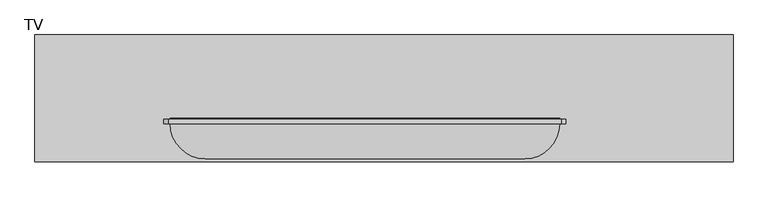
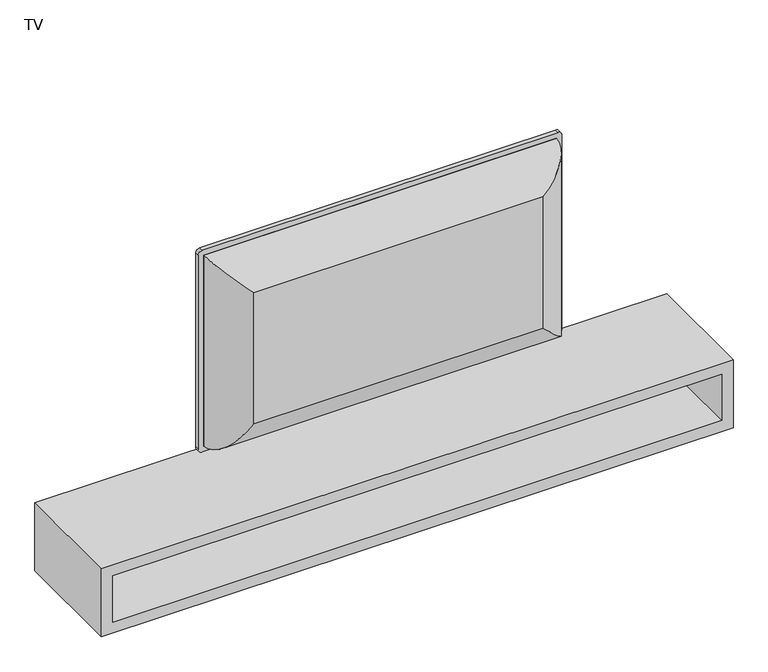
"""IFC4 building model written with IfcOpenShell, lengths in millimetres: furniture geometry, BA_Floathing TV shelf : TV."""

from ifc_helpers import new_model, si_unit, point, frame, frame_2d, origin, place, context, project, spatial, polyline, circle_curve, ellipse_curve, trimmed, segment, composite_curve, outline, extrude, faceted_brep, source, transform, mapped, element, save
from ifc_brep_helpers import plane_surface, cylinder_surface, advanced_brep


def tv_c5042563(model_context):
    return source(origin(), model_context, "Body", "SolidModel", [
        faceted_brep([(-488.4382596, 288.0, 1482.6751733), (738.4382596, 288.0, 1482.6751733), (738.4382596, 288.0, 780.0), (-488.4382596, 288.0, 780.0), (678.4382596, 288.0, 1442.6751733), (-428.4382596, 288.0, 1442.6751733), (-428.4382596, 288.0, 820.0), (678.4382596, 288.0, 820.0), (-488.4382596, 270.0, 1482.6751733), (-488.4382596, 270.0, 780.0), (738.4382596, 270.0, 780.0), (738.4382596, 270.0, 1482.6751733), (678.4382596, 285.0, 1442.6751733), (678.4382596, 285.0, 820.0), (-428.4382596, 285.0, 820.0), (-428.4382596, 285.0, 1442.6751733)], [[[0, 1, 2, 3], [4, 5, 6, 7]], [[8, 9, 10, 11]], [[1, 0, 8, 11]], [[2, 1, 11, 10]], [[3, 2, 10, 9]], [[0, 3, 9, 8]], [[12, 13, 14, 15]], [[12, 15, 5, 4]], [[15, 14, 6, 5]], [[14, 13, 7, 6]], [[13, 12, 4, 7]]]),
        extrude(outline(composite_curve([segment(trimmed(circle_curve(frame_2d((1487.6751733, -493.4382596)), 15.0), [point((1502.6751733, -493.4382596))], [point((1487.6751733, -508.4382596))], False, "CARTESIAN"), True, "CONTINUOUS"), segment(polyline([(1487.6751733, -508.4382596), (775.0, -508.4382596)]), True, "CONTINUOUS"), segment(trimmed(circle_curve(frame_2d((775.0, -493.4382596)), 15.0), [point((775.0, -508.4382596))], [point((760.0, -493.4382596))], False, "CARTESIAN"), True, "CONTINUOUS"), segment(polyline([(760.0, -493.4382596), (760.0, 743.4382596)]), True, "CONTINUOUS"), segment(trimmed(circle_curve(frame_2d((775.0, 743.4382596)), 15.0), [point((760.0, 743.4382596))], [point((775.0, 758.4382596))], False, "CARTESIAN"), True, "CONTINUOUS"), segment(polyline([(775.0, 758.4382596), (1487.6751733, 758.4382596)]), True, "CONTINUOUS"), segment(trimmed(circle_curve(frame_2d((1487.6751733, 743.4382596)), 15.0), [point((1487.6751733, 758.4382596))], [point((1502.6751733, 743.4382596))], False, "CARTESIAN"), True, "CONTINUOUS"), segment(polyline([(1502.6751733, 743.4382596), (1502.6751733, -493.4382596)]), True, "CONTINUOUS")], self_intersect=False), holes=[polyline([(1482.6751733, -488.4382596), (1482.6751733, 738.4382596), (780.0, 738.4382596), (780.0, -488.4382596), (1482.6751733, -488.4382596)])]), frame((0.0, 270.0, 0.0), z_axis=(0.0, 1.0, 0.0), x_axis=(0.0, 0.0, 1.0)), (0.0, 0.0, 1.0), 15.0),
        advanced_brep(
        [(-488.4382596, 270.0, 780.0), (-488.4382596, 270.0, 1482.6751733), (738.4382596, 270.0, 1482.6751733), (738.4382596, 270.0, 780.0), (-378.4382596, 160.0, 1372.6751733), (-378.4382596, 160.0, 890.0), (628.4382596, 160.0, 890.0), (628.4382596, 160.0, 1372.6751733)],
        [
            (0, 1),
            (1, 2),
            (2, 3),
            (3, 0),
            (4, 5),
            (5, 6),
            (6, 7),
            (7, 4),
            (0, 5, ellipse_curve(frame((-378.4382596, 270.0, 890.0), z_axis=(-0.7071067811865475, 0.0, 0.7071067811865475), x_axis=(0.7071067811865474, 0.0, 0.7071067811865476)), 155.5634919, 110.0)),
            (4, 1, ellipse_curve(frame((-378.4382596, 270.0, 1372.6751733), z_axis=(-0.7071067811865475, 0.0, -0.7071067811865475), x_axis=(-0.7071067811865474, 0.0, 0.7071067811865476)), 155.5634919, 110.0)),
            (7, 2, ellipse_curve(frame((628.4382596, 270.0, 1372.6751733), z_axis=(-0.7071067811865475, 0.0, 0.7071067811865475), x_axis=(0.7071067811865476, 0.0, 0.7071067811865474)), 155.5634919, 110.0)),
            (6, 3, ellipse_curve(frame((628.4382596, 270.0, 890.0), z_axis=(0.7071067811865475, 0.0, 0.7071067811865475), x_axis=(0.7071067811865474, 0.0, -0.7071067811865476)), 155.5634919, 110.0)),
        ],
        [
            plane_surface(frame((738.4382596, 270.0, 1482.6751733), z_axis=(0.0, 1.0, 0.0), x_axis=(1.0, 0.0, 0.0))),
            plane_surface(frame((738.4382596, 160.0, 1482.6751733), z_axis=(0.0, -1.0, 0.0), x_axis=(-1.0, 0.0, 0.0))),
            cylinder_surface(frame((-378.4382596, 270.0, 780.0), z_axis=(0.0, 0.0, 1.0), x_axis=(-1.0, 0.0, 0.0)), 110.0),
            cylinder_surface(frame((-488.4382596, 270.0, 1372.6751733), z_axis=(1.0, 0.0, 0.0), x_axis=(0.0, 0.0, 1.0)), 110.0),
            cylinder_surface(frame((628.4382596, 270.0, 1482.6751733), z_axis=(0.0, 0.0, -1.0), x_axis=(1.0, 0.0, 0.0)), 110.0),
            cylinder_surface(frame((738.4382596, 270.0, 890.0), z_axis=(-1.0, 0.0, 0.0), x_axis=(0.0, 0.0, -1.0)), 110.0),
        ],
        [
            (0, [[1, 2, 3, 4]]),
            (1, [[5, 6, 7, 8]]),
            (2, [[9, -5, 10, -1]]),
            (3, [[-10, -8, 11, -2]]),
            (4, [[12, -3, -11, -7]]),
            (5, [[-9, -4, -12, -6]]),
        ],
    ),
        extrude(outline(polyline([(550.0, -915.0), (300.0, -915.0), (300.0, 1285.0), (550.0, 1285.0), (550.0, -915.0)]), holes=[polyline([(510.0, -875.0), (510.0, 1245.0), (340.0, 1245.0), (340.0, -875.0), (510.0, -875.0)])]), frame((0.0, 150.0, 0.0), z_axis=(0.0, 1.0, 0.0), x_axis=(0.0, 0.0, 1.0)), (0.0, 0.0, 1.0), 400.0),
    ])


if __name__ == "__main__":
    model = new_model("IFC4")
    model_context = context("Model", 3, world=origin())
    ifc_project = project(units=[si_unit("LENGTHUNIT", "METRE", prefix="MILLI")], contexts=[model_context])
    site = spatial("IfcSite", under=ifc_project)
    building = spatial("IfcBuilding", under=site)
    placement = place(None, origin())
    tv_shape = tv_c5042563(model_context)
    element("IfcFurniture", 1, ObjectType="BA_Floathing TV shelf : TV", at=placement, inside=building, context=model_context, shape_type="MappedRepresentation", body=[
        mapped(tv_shape, transform((0.0, 0.0, 0.0), x_axis=(1.0, 0.0, 0.0), y_axis=(0.0, 1.0, 0.0), z_axis=(0.0, 0.0, 1.0))),
    ])
    save(model, "model.ifc")

# Revit data of these elements
# Type "BA_Floathing TV shelf : TV"
#   TV position [instance default] = 1160 mm
#   Shelf lenght [instance default] = 2200 mm
#   Default Elevation = 0
# Element 1 (IfcFurniture, "BA_Floathing TV shelf : TV")
#   Materials on its faces: "Default", "TV - Glass", "TV - Screen"
# Materials
#   "Default": class "Generic", colour RGB 255 255 255, transparency 0, Cost = 0
#   "TV - Glass": class "Miscellaneous", colour RGB 157 157 157, transparency 0.9
#   "TV - Screen": class "Miscellaneous", colour RGB 0 0 0, transparency 0
